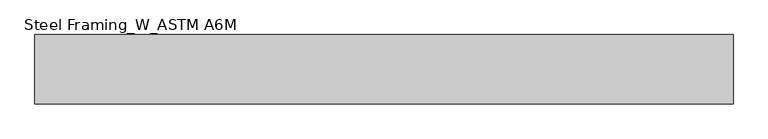
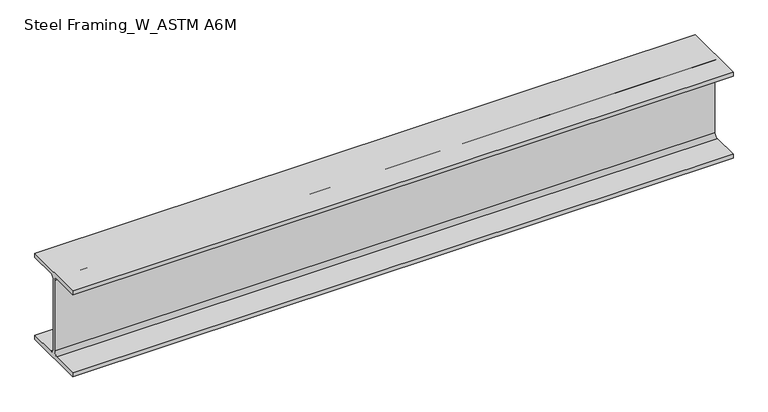
"""IFC4 building model written with IfcOpenShell, lengths in millimetres: beam geometry, Steel Framing_W_ASTM A6M : H_SB_AR_S02_W360x91_B3."""

import ifcopenshell
import ifcopenshell.guid

model = None  # the IFC model being written
_history = None  # IfcOwnerHistory: only IFC2X3 demands one
_inside = {}  # id of a spatial element -> (the spatial element, [elements in it])
_under = {}  # id of a project, library or spatial element -> (it, [spatial elements below it])
_declared = {}  # id of a project -> (the project, [libraries it declares])
_typed = {}  # id of a type object -> (the type object, [elements of that type])
_made_of = {}  # id of a material, layer set ... -> (it, [elements and type objects made of it])


def new_model(schema):
    """Start an empty IFC model of exactly this schema.

    Asked for "IFC4X3", IfcOpenShell would pick the latest addendum, in which some entities
    have other attributes; the version numbers below select the first issue.
    IFC2X3 requires an IfcOwnerHistory on every rooted entity: one is made here for all.
    """
    global model, _history
    if schema == "IFC4X3":
        model = ifcopenshell.file(schema_version=(4, 3, 0, 0))
    else:
        model = ifcopenshell.file(schema=schema)
    _inside.clear()
    _under.clear()
    _declared.clear()
    _typed.clear()
    _made_of.clear()
    _history = None
    if model.schema == "IFC2X3":
        org = make("IfcOrganization", Name="unknown")
        user = make(
            "IfcPersonAndOrganization",
            ThePerson=make("IfcPerson", FamilyName="unknown"),
            TheOrganization=org,
        )
        app = make(
            "IfcApplication",
            ApplicationDeveloper=org,
            Version="unknown",
            ApplicationFullName="unknown",
            ApplicationIdentifier="unknown",
        )
        _history = make(
            "IfcOwnerHistory",
            OwningUser=user,
            OwningApplication=app,
            ChangeAction="ADDED",
            CreationDate=0,
        )
    return model


def make(cls, **values):
    """One entity of the class cls with the attributes given. An attribute that is None is left unset."""
    return model.create_entity(
        cls, **{name: value for name, value in values.items() if value is not None}
    )


def rooted(cls, **values):
    """An entity with a GlobalId (a new one), such as an element, a storey or a relation."""
    return make(cls, GlobalId=ifcopenshell.guid.new(), OwnerHistory=_history, **values)


def si_unit(unit_type, name, prefix=None):
    """IfcSIUnit, for example si_unit("LENGTHUNIT", "METRE", prefix="MILLI")."""
    return make("IfcSIUnit", UnitType=unit_type, Prefix=prefix, Name=name)


def assignment(units):
    """IfcUnitAssignment: the units of a project."""
    return None if units is None else make("IfcUnitAssignment", Units=units)


def point(xyz):
    """IfcCartesianPoint."""
    return None if xyz is None else make("IfcCartesianPoint", Coordinates=xyz)


def direction(xyz):
    """IfcDirection."""
    return None if xyz is None else make("IfcDirection", DirectionRatios=xyz)


def frame(location, z_axis=None, x_axis=None):
    """IfcAxis2Placement3D, a coordinate frame: its origin and axes. An axis left out is left unset."""
    return make(
        "IfcAxis2Placement3D",
        Location=point(location),
        Axis=direction(z_axis),
        RefDirection=direction(x_axis),
    )


def frame_2d(location, x_axis=None):
    """IfcAxis2Placement2D, a coordinate frame in the plane: its origin and x axis."""
    return make(
        "IfcAxis2Placement2D", Location=point(location), RefDirection=direction(x_axis)
    )


def origin():
    """The frame at (0, 0, 0) with its axes left unset."""
    return frame((0.0, 0.0, 0.0))


def place(relative_to, where):
    """IfcLocalPlacement: puts the frame where relative to a parent placement (None: the world)."""
    return make(
        "IfcLocalPlacement", PlacementRelTo=relative_to, RelativePlacement=where
    )


def context(
    kind, dimensions, precision=None, world=None, true_north=None, identifier=None
):
    """IfcGeometricRepresentationContext, for example the 3D "Model" context."""
    return make(
        "IfcGeometricRepresentationContext",
        ContextIdentifier=identifier,
        ContextType=kind,
        CoordinateSpaceDimension=dimensions,
        Precision=precision,
        WorldCoordinateSystem=world,
        TrueNorth=true_north,
    )


def project(units=None, contexts=None):
    """IfcProject with its units and contexts."""
    return rooted(
        "IfcProject",
        Name="project",
        RepresentationContexts=contexts,
        UnitsInContext=assignment(units),
    )


def spatial(cls, under=None, at=None, **own):
    """A site, building, storey or space (cls), placed at a placement, below another one or the project."""
    s = rooted(cls, ObjectPlacement=at, **own)
    if under is not None:
        _under.setdefault(under.id(), (under, []))[1].append(s)
    return s


def polyline(points):
    """IfcPolyline through the points."""
    return make("IfcPolyline", Points=[point(p) for p in points])


def circle_curve(where, radius):
    """IfcCircle in the frame where."""
    return make("IfcCircle", Position=where, Radius=radius)


def trimmed(basis, trim1, trim2, sense, master):
    """IfcTrimmedCurve: the piece of a basis curve between two trims."""
    return make(
        "IfcTrimmedCurve",
        BasisCurve=basis,
        Trim1=trim1,
        Trim2=trim2,
        SenseAgreement=sense,
        MasterRepresentation=master,
    )


def segment(curve, same_sense, transition):
    """IfcCompositeCurveSegment."""
    return make(
        "IfcCompositeCurveSegment",
        Transition=transition,
        SameSense=same_sense,
        ParentCurve=curve,
    )


def composite_curve(segments, self_intersect=None):
    """IfcCompositeCurve: segments joined end to end."""
    return make("IfcCompositeCurve", Segments=segments, SelfIntersect=self_intersect)


def outline(outer, holes=None, kind="AREA"):
    """IfcArbitraryClosedProfileDef: a profile drawn as a closed curve; with holes, ...WithVoids."""
    if holes is None:
        return make("IfcArbitraryClosedProfileDef", ProfileType=kind, OuterCurve=outer)
    return make(
        "IfcArbitraryProfileDefWithVoids",
        ProfileType=kind,
        OuterCurve=outer,
        InnerCurves=holes,
    )


def extrude(swept, where, along, depth):
    """IfcExtrudedAreaSolid: the profile swept, set in the frame where, extruded along a direction by depth."""
    return make(
        "IfcExtrudedAreaSolid",
        SweptArea=swept,
        Position=where,
        ExtrudedDirection=direction(along),
        Depth=depth,
    )


def shape(context_of_items, identifier, shape_type, items):
    """IfcShapeRepresentation: the items that make up one representation, for example the "Body"."""
    return make(
        "IfcShapeRepresentation",
        ContextOfItems=context_of_items,
        RepresentationIdentifier=identifier,
        RepresentationType=shape_type,
        Items=items,
    )


def source(mapping_origin, context_of_items, identifier, shape_type, items):
    """IfcRepresentationMap: a shape defined once, which mapped items show again and again."""
    return make(
        "IfcRepresentationMap",
        MappingOrigin=mapping_origin,
        MappedRepresentation=shape(context_of_items, identifier, shape_type, items),
    )


def transform(
    local_origin,
    x_axis=None,
    y_axis=None,
    z_axis=None,
    scale=None,
    scale2=None,
    scale3=None,
    uniform=True,
):
    """IfcCartesianTransformationOperator3D, or its non-uniform kind. x_axis, y_axis, z_axis: its Axis1, 2, 3."""
    if uniform:
        return make(
            "IfcCartesianTransformationOperator3D",
            Axis1=direction(x_axis),
            Axis2=direction(y_axis),
            LocalOrigin=point(local_origin),
            Scale=scale,
            Axis3=direction(z_axis),
        )
    return make(
        "IfcCartesianTransformationOperator3DnonUniform",
        Axis1=direction(x_axis),
        Axis2=direction(y_axis),
        LocalOrigin=point(local_origin),
        Scale=scale,
        Axis3=direction(z_axis),
        Scale2=scale2,
        Scale3=scale3,
    )


def mapped(mapping_source, mapping_target):
    """IfcMappedItem: shows the shape of a source again, moved by a transform."""
    return make(
        "IfcMappedItem", MappingSource=mapping_source, MappingTarget=mapping_target
    )


def made_of(thing, what):
    """Note that an element or type object is made of a material, layer set ...; save() writes the relation."""
    if what is not None:
        _made_of.setdefault(what.id(), (what, []))[1].append(thing)
    return thing


def element(
    cls,
    number,
    at=None,
    inside=None,
    cuts=None,
    type_object=None,
    material=None,
    context=None,
    identifier="Body",
    shape_type=None,
    held_by="IfcProductDefinitionShape",
    body=None,
    shapes=None,
    **own,
):
    """One element of the class cls, such as IfcWall. Its Tag is "e" and its number.

    at: its placement. inside: the storey or other place that contains it. cuts: it is an
    opening in that element (IfcRelVoidsElement). A single representation is given by context,
    identifier, shape_type and body (its items); several are given by shapes. held_by: the class
    of the entity that holds the representations. save() writes the other relations.
    """
    e = rooted(cls, Tag="e%d" % number, ObjectPlacement=at, **own)
    if body is not None:
        shapes = [shape(context, identifier, shape_type, body)]
    if shapes is not None:
        e.Representation = make(held_by, Representations=shapes)
    if inside is not None:
        _inside.setdefault(inside.id(), (inside, []))[1].append(e)
    if cuts is not None:
        rooted(
            "IfcRelVoidsElement", RelatingBuildingElement=cuts, RelatedOpeningElement=e
        )
    if type_object is not None:
        _typed.setdefault(type_object.id(), (type_object, []))[1].append(e)
    return made_of(e, material)


def aggregate(whole, parts):
    """IfcRelAggregates: a whole, such as a stair, and the parts it consists of."""
    return rooted("IfcRelAggregates", RelatingObject=whole, RelatedObjects=parts)


def save(model, path):
    """Write the relations noted so far, then the file.

    IfcRelAggregates (storeys below a building ...), IfcRelContainedInSpatialStructure (elements
    in a storey), IfcRelDefinesByType, IfcRelAssociatesMaterial and IfcRelDeclares: one each for
    every whole, place, type object, material and project.
    """
    for whole, parts in _under.values():
        aggregate(whole, parts)
    for where, things in _inside.values():
        rooted(
            "IfcRelContainedInSpatialStructure",
            RelatedElements=things,
            RelatingStructure=where,
        )
    for kind, things in _typed.values():
        rooted("IfcRelDefinesByType", RelatedObjects=things, RelatingType=kind)
    for what, things in _made_of.values():
        rooted("IfcRelAssociatesMaterial", RelatedObjects=things, RelatingMaterial=what)
    for by, libraries in _declared.values():
        rooted("IfcRelDeclares", RelatingContext=by, RelatedDefinitions=libraries)
    model.write(path)


def steel_framing_w_astm_a6m_a9de8b5d(model_context):
    return source(origin(), model_context, "Body", "SweptSolid", [
        extrude(outline(composite_curve([segment(polyline([(127.0, -160.1), (127.0, -176.5), (-127.0, -176.5), (-127.0, -160.1), (-19.865, -160.1)]), True, "CONTINUOUS"), segment(trimmed(circle_curve(frame_2d((-19.865, -145.0)), 15.1), [point((-19.865, -160.1))], [point((-4.765, -145.0))], True, "CARTESIAN"), True, "CONTINUOUS"), segment(polyline([(-4.765, -145.0), (-4.765, 145.0)]), True, "CONTINUOUS"), segment(trimmed(circle_curve(frame_2d((-19.865, 145.0)), 15.1), [point((-4.765, 145.0))], [point((-19.865, 160.1))], True, "CARTESIAN"), True, "CONTINUOUS"), segment(polyline([(-19.865, 160.1), (-127.0, 160.1), (-127.0, 176.5), (127.0, 176.5), (127.0, 160.1), (19.865, 160.1)]), True, "CONTINUOUS"), segment(trimmed(circle_curve(frame_2d((19.865, 145.0)), 15.1), [point((19.865, 160.1))], [point((4.765, 145.0))], True, "CARTESIAN"), True, "CONTINUOUS"), segment(polyline([(4.765, 145.0), (4.765, -145.0)]), True, "CONTINUOUS"), segment(trimmed(circle_curve(frame_2d((19.865, -145.0)), 15.1), [point((4.765, -145.0))], [point((19.865, -160.1))], True, "CARTESIAN"), True, "CONTINUOUS"), segment(polyline([(19.865, -160.1), (127.0, -160.1)]), True, "CONTINUOUS")], self_intersect=False)), frame((-1203.3, 0.0, 0.0), z_axis=(1.0, 0.0, 0.0), x_axis=(0.0, 1.0, 0.0)), (0.0, 0.0, 1.0), 2563.6),
    ])


if __name__ == "__main__":
    model = new_model("IFC4")
    model_context = context("Model", 3, world=origin())
    ifc_project = project(units=[si_unit("LENGTHUNIT", "METRE", prefix="MILLI")], contexts=[model_context])
    site = spatial("IfcSite", under=ifc_project)
    building = spatial("IfcBuilding", under=site)
    placement = place(None, origin())
    steel_framing_w_astm_a6m_shape = steel_framing_w_astm_a6m_a9de8b5d(model_context)
    element("IfcBeam", 1, ObjectType="Steel Framing_W_ASTM A6M : H_SB_AR_S02_W360x91_B3", at=placement, inside=building, context=model_context, shape_type="MappedRepresentation", body=[
        mapped(steel_framing_w_astm_a6m_shape, transform((0.0, 0.0, 0.0), x_axis=(1.0, 0.0, 0.0), y_axis=(0.0, 1.0, 0.0), z_axis=(0.0, 0.0, 1.0))),
    ])
    save(model, "model.ifc")

# Revit data of these elements
# Type "Steel Framing_W_ASTM A6M : H_SB_AR_S02_W360x91_B3"
#   Type Mark = "B3"
#   Section Name Key = "W14x61"
#   Width = 25.4 cm
#   Web Thickness = 0.953 cm
#   Web Fillet = 1.51 cm
#   Warping Constant = 1260000.0 cm⁶
#   Torsional Moment of Inertia = 91.20 cm⁴
#   Section Area = 115.0 cm²
#   Plastic Modulus weak axis = 537.0 cm³
#   Plastic Modulus strong axis = 1670.0 cm³
#   Perimeter = 1.68 m²/m
#   Nominal Weight = 91.00 kgf/m
#   Moment of Inertia weak axis = 4450.00 cm⁴
#   Moment of Inertia strong axis = 26600.00 cm⁴
#   Height = 35.3 cm
#   Flange Thickness = 1.64 cm
#   Elastic Modulus weak axis = 352.0 cm³
#   Elastic Modulus strong axis = 1510.0 cm³
#   Centroid Vertical = 17.65 cm
#   Centroid Horizontal = 12.7 cm
#   Length [instance default] = 1500 mm
#   Structural Material [instance default] = Steel, 45-345
#   Bolt Spacing = 0
#   Assembly Code = ""
# Element 1 (IfcBeam, "Steel Framing_W_ASTM A6M : H_SB_AR_S02_W360x91_B3")
#   Materials on its faces: "Steel, 45-345"
# Materials
#   "Steel, 45-345": class "Metal", colour RGB 189 187 185, transparency 0, Description = "Steel 345 MPa", Cost = 0
